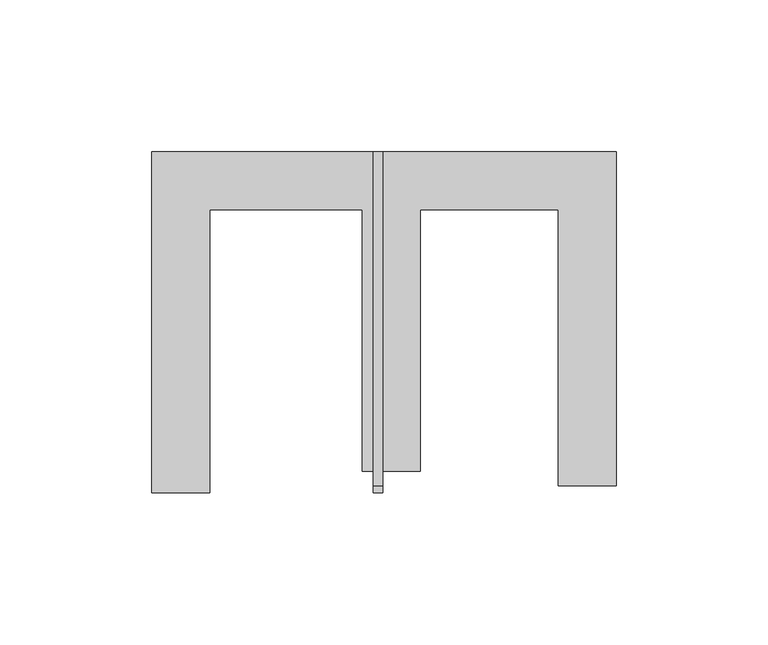
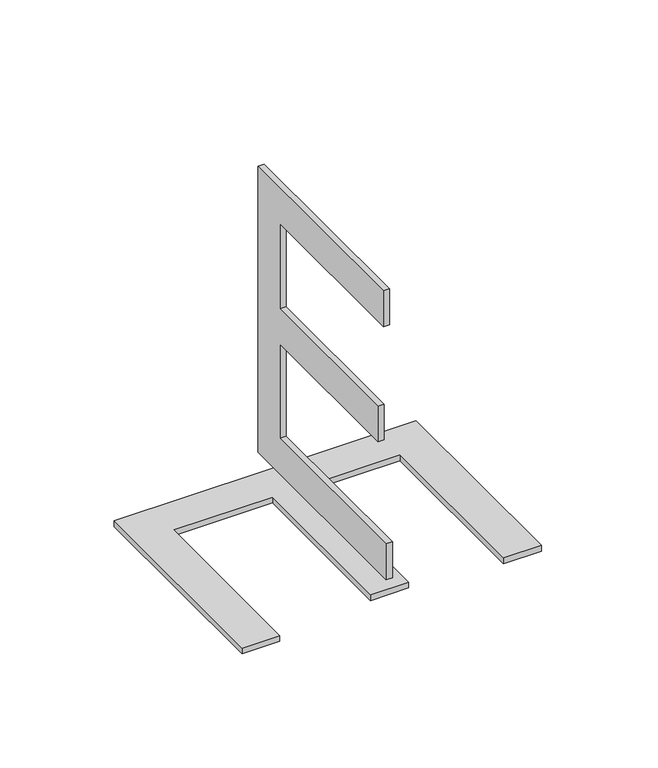
"""IFC4 building model written with IfcOpenShell, lengths in millimetres: proxy geometry, Grid Number2_FedEx : Grid Number2_FedEx."""

from ifc_helpers import new_model, si_unit, frame, origin, origin_with_axes, place, context, project, spatial, polyline, outline, extrude, source, transform, mapped, element, save


def entourage_0ddd790d(model_context):
    return source(origin(), model_context, "Body", "SweptSolid", [
        extrude(outline(polyline([(-184.2739267, 276.3432839), (-31.1785101, 276.3432839), (-31.1785101, 166.3059532), (-50.3154372, 166.3059532), (-50.3154372, 257.2063569), (-95.765639, 257.2063569), (-95.765639, 171.090185), (-114.9025661, 171.090185), (-114.9025661, 257.2063569), (-165.1369997, 257.2063569), (-165.1369997, 163.9138373), (-184.2739267, 163.9138373), (-184.2739267, 276.3432839)])), origin_with_axes(), (0.0, 0.0, 1.0), 3.175),
        extrude(outline(polyline([(276.3432839, 14.2382753), (163.9138373, 14.2382753), (163.9138373, 33.3752024), (257.2063569, 33.3752024), (257.2063569, 83.609636), (171.090185, 83.609636), (171.090185, 102.7465631), (257.2063569, 102.7465631), (257.2063569, 148.1967649), (166.3059532, 148.1967649), (166.3059532, 167.333692), (276.3432839, 167.333692), (276.3432839, 14.2382753)])), frame((-111.2489267, 0.0, 0.0), z_axis=(1.0, 0.0, 0.0), x_axis=(0.0, 1.0, 0.0)), (0.0, 0.0, 1.0), 3.175),
    ])


if __name__ == "__main__":
    model = new_model("IFC4")
    model_context = context("Model", 3, world=origin())
    ifc_project = project(units=[si_unit("LENGTHUNIT", "METRE", prefix="MILLI")], contexts=[model_context])
    site = spatial("IfcSite", under=ifc_project)
    building = spatial("IfcBuilding", under=site)
    placement = place(None, origin())
    entourage_shape = entourage_0ddd790d(model_context)
    element("IfcBuildingElementProxy", 1, Name="Grid Number2_FedEx : Grid Number2_FedEx", ObjectType="Grid Number2_FedEx : Grid Number2_FedEx", at=placement, inside=building, context=model_context, shape_type="MappedRepresentation", body=[
        mapped(entourage_shape, transform((0.0, 0.0, 0.0), x_axis=(1.0, 0.0, 0.0), y_axis=(0.0, 1.0, 0.0), z_axis=(0.0, 0.0, 1.0))),
    ])
    save(model, "model.ifc")

# Revit data of these elements
# Type "Grid Number2_FedEx : Grid Number2_FedEx"
#   Grid [instance default] = "S"
#   Label Width [instance default] = 1' - 0"
#   Half Box Width2 [instance default] = 0' - 6.13846"
#   Half Box Width [instance default] = 0' - 6"
#   Robust [instance default] = yes
#   Height = 0
#   Assembly Code = ""
# Element 1 (IfcBuildingElementProxy, "Grid Number2_FedEx : Grid Number2_FedEx")
#   Grid = "E"
#   Robust = no
#   Materials on its faces: "Letter"
# Materials
#   "Letter": class "Unassigned", colour RGB 178 187 30, transparency 0, Comments = "Rendering appearance not upgraded "
